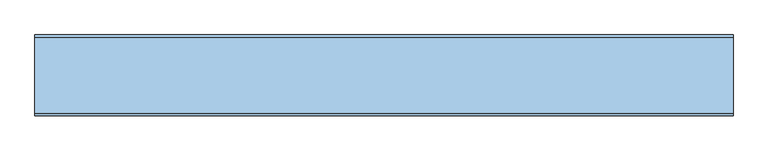
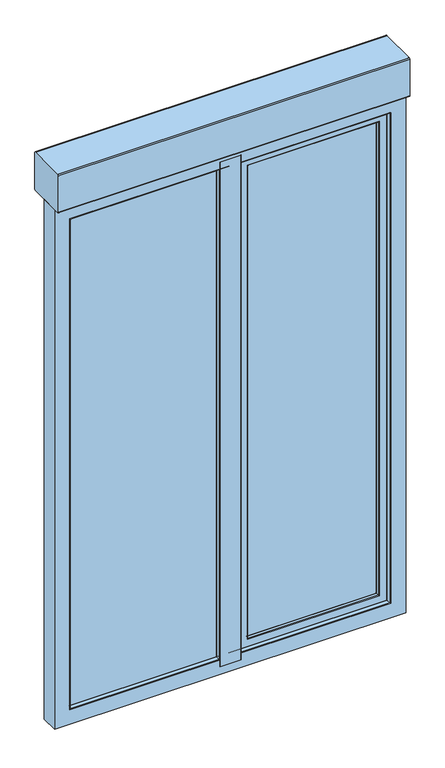
"""IFC4 building model written with IfcOpenShell, lengths in millimetres: window geometry, 2019_ES_Ventana_Replus_re80pvc301_11103_box_1-Hoja_Panel-Fijo-Lateral_con-Compacto : Ventana Sala Oeste."""

from ifc_helpers import new_model, si_unit, point, frame, frame_2d, origin, place, context, project, spatial, polyline, circle_curve, ellipse_curve, trimmed, segment, composite_curve, outline, extrude, source, transform, mapped, element, save
from ifc_brep_helpers import plane_surface, cylinder_surface, advanced_brep


def window_1332a1be(model_context):
    return source(origin(), model_context, "Body", "SolidModel", [
        extrude(outline(composite_curve([segment(trimmed(circle_curve(frame_2d((-55.0, 3315.0)), 5.0), [point((-55.0, 3310.0))], [point((-60.0, 3315.0))], False, "CARTESIAN"), True, "CONTINUOUS"), segment(polyline([(-60.0, 3315.0), (-60.0, 3490.0)]), True, "CONTINUOUS"), segment(trimmed(circle_curve(frame_2d((-55.0, 3490.0)), 5.0), [point((-60.0, 3490.0))], [point((-55.0, 3495.0))], False, "CARTESIAN"), True, "CONTINUOUS"), segment(polyline([(-55.0, 3495.0), (120.0, 3495.0)]), True, "CONTINUOUS"), segment(trimmed(circle_curve(frame_2d((120.0, 3490.0)), 5.0), [point((120.0, 3495.0))], [point((125.0, 3490.0))], False, "CARTESIAN"), True, "CONTINUOUS"), segment(polyline([(125.0, 3490.0), (125.0, 3315.0)]), True, "CONTINUOUS"), segment(trimmed(circle_curve(frame_2d((120.0, 3315.0)), 5.0), [point((125.0, 3315.0))], [point((120.0, 3310.0))], False, "CARTESIAN"), True, "CONTINUOUS"), segment(polyline([(120.0, 3310.0), (-55.0, 3310.0)]), True, "CONTINUOUS")], self_intersect=False)), frame((-800.0, 0.0, 0.0), z_axis=(1.0, 0.0, 0.0), x_axis=(0.0, 1.0, 0.0)), (0.0, 0.0, 1.0), 1600.0),
        extrude(outline(polyline([(78.4999991, 1470.0), (118.4999991, 1470.0), (118.4999991, 1360.0), (98.4999991, 1360.0), (98.4999991, 1450.0), (78.4999991, 1450.0), (78.4999991, 1470.0)])), frame((38.5, 0.0, 0.0), z_axis=(1.0, 0.0, 0.0), x_axis=(0.0, 1.0, 0.0)), (0.0, 0.0, 1.0), 12.0),
        extrude(outline(polyline([(58.7312385, 78.4999991), (58.7312385, 68.4999991), (30.2687615, 68.4999991), (30.2687615, 78.4999991), (58.7312385, 78.4999991)])), frame((0.0, 0.0, 1435.217127), z_axis=(0.0, 0.0, 1.0), x_axis=(1.0, 0.0, 0.0)), (0.0, 0.0, 1.0), 49.565746),
        extrude(outline(polyline([(-37.0063666, -11.4999962), (-734.1891471, -11.4999962), (-734.1891471, -7.4999962), (-37.0063666, -7.4999962), (-37.0063666, -11.4999962)])), frame((0.0, 0.0, 875.6108529), z_axis=(0.0, 0.0, 1.0), x_axis=(1.0, 0.0, 0.0)), (0.0, 0.0, 1.0), 2368.7782941),
        extrude(outline(polyline([(-37.0063666, 6.5), (-734.1891471, 6.5), (-734.1891471, 10.5), (-37.0063666, 10.5), (-37.0063666, 6.5)])), frame((0.0, 0.0, 875.6108529), z_axis=(0.0, 0.0, 1.0), x_axis=(1.0, 0.0, 0.0)), (0.0, 0.0, 1.0), 2368.7782941),
        extrude(outline(polyline([(-37.0063666, 24.4999997), (-734.1891471, 24.4999997), (-734.1891471, 28.4999997), (-37.0063666, 28.4999997), (-37.0063666, 24.4999997)])), frame((0.0, 0.0, 875.6108529), z_axis=(0.0, 0.0, 1.0), x_axis=(1.0, 0.0, 0.0)), (0.0, 0.0, 1.0), 2368.7782941),
        advanced_brep(
        [(-22.1502489, 49.9816666, 3264.0497511), (-22.1502489, 49.9816666, 855.9502489), (-41.8192398, 49.2838062, 875.6192398), (-41.8192398, 49.2838062, 3244.3807602), (-46.4697163, 45.5846502, 880.2697163), (-46.4697163, 45.5846502, 3239.7302837), (-754.0497503, 49.9816666, 855.9502489), (-734.3807594, 49.2838062, 875.6192398), (-21.0, 48.871505, 3265.2), (-21.0, 48.871505, 854.8), (-51.0475336, 28.5000036, 884.8475336), (-51.0475336, 28.5000036, 3235.1524664), (-729.7302829, 45.5846502, 880.2697163), (-43.2922784, 28.5000036, 877.0922784), (-43.2922784, 28.5000036, 3242.9077216), (-732.9077208, 28.5000036, 3242.9077216), (-732.9077208, 28.5000036, 877.0922784), (-725.1524657, 28.5000036, 884.8475336), (-725.1524657, 28.5000036, 3235.1524664), (-35.4855, 36.306782, 869.2855), (-35.4855, 36.306782, 3250.7145), (-35.4855, 39.5069121, 869.2855), (-35.4855, 39.5069121, 3250.7145), (-740.7144993, 36.306782, 869.2855), (-21.0, 39.5069121, 854.8), (-21.0, 39.5069121, 3265.2), (-755.1999993, 39.5069121, 3265.2), (-755.1999993, 39.5069121, 854.8), (-740.7144993, 39.5069121, 869.2855), (-740.7144993, 39.5069121, 3250.7145), (-755.1999993, 48.871505, 854.8), (-754.0497503, 49.9816666, 3264.0497511), (-734.3807594, 49.2838062, 3244.3807602), (-729.7302829, 45.5846502, 3239.7302837), (-740.7144993, 36.306782, 3250.7145), (-755.1999993, 48.871505, 3265.2)],
        [
            (0, 1),
            (1, 2),
            (2, 3),
            (3, 0),
            (2, 4, ellipse_curve(frame((-41.6449168, 44.2918491, 875.4449168), z_axis=(0.7071067811865475, 0.0, 0.7071067811865475), x_axis=(-0.7071067811865474, 0.0, 0.7071067811865476)), 7.0639967, 4.995)),
            (4, 5),
            (5, 3, ellipse_curve(frame((-41.6449168, 44.2918491, 3244.5550832), z_axis=(0.7071067811865475, 0.0, -0.7071067811865475), x_axis=(0.7071067811865474, 0.0, 0.7071067811865476)), 7.0639967, 4.995)),
            (1, 6),
            (6, 7),
            (7, 2),
            (8, 9),
            (9, 1, ellipse_curve(frame((-22.1108601, 48.871505, 855.9108601), z_axis=(0.7071067811865475, 0.0, 0.7071067811865475), x_axis=(-0.7071067811865474, 0.0, 0.7071067811865476)), 1.5709935, 1.1108601)),
            (0, 8, ellipse_curve(frame((-22.1108601, 48.871505, 3264.0891399), z_axis=(0.7071067811865475, 0.0, -0.7071067811865475), x_axis=(0.7071067811865474, 0.0, 0.7071067811865476)), 1.5709935, 1.1108601)),
            (4, 10),
            (10, 11),
            (11, 5),
            (7, 12, ellipse_curve(frame((-734.5550824, 44.2918491, 875.4449168), z_axis=(0.7071067811865475, 0.0, -0.7071067811865475), x_axis=(0.7071067811865476, 0.0, 0.7071067811865474)), 7.0639967, 4.995)),
            (12, 4),
            (13, 14),
            (14, 15),
            (15, 16),
            (16, 13),
            (10, 17),
            (17, 18),
            (18, 11),
            (12, 17),
            (13, 19),
            (19, 20),
            (20, 14),
            (19, 21),
            (21, 22),
            (22, 20),
            (16, 23),
            (23, 19),
            (24, 25),
            (25, 26),
            (26, 27),
            (27, 24),
            (21, 28),
            (28, 29),
            (29, 22),
            (23, 28),
            (8, 25),
            (24, 9),
            (27, 30),
            (30, 9),
            (30, 6, ellipse_curve(frame((-754.0891391, 48.871505, 855.9108601), z_axis=(0.7071067811865475, 0.0, -0.7071067811865475), x_axis=(0.7071067811865476, 0.0, 0.7071067811865474)), 1.5709935, 1.1108601)),
            (6, 31),
            (31, 32),
            (32, 7),
            (32, 33, ellipse_curve(frame((-734.5550824, 44.2918491, 3244.5550832), z_axis=(-0.7071067811865475, 0.0, -0.7071067811865475), x_axis=(0.7071067811865474, 0.0, -0.7071067811865476)), 7.0639967, 4.995)),
            (33, 12),
            (33, 18),
            (15, 34),
            (34, 23),
            (34, 29),
            (26, 35),
            (35, 30),
            (35, 31, ellipse_curve(frame((-754.0891391, 48.871505, 3264.0891399), z_axis=(-0.7071067811865475, 0.0, -0.7071067811865475), x_axis=(0.7071067811865474, 0.0, -0.7071067811865476)), 1.5709935, 1.1108601)),
            (31, 0),
            (3, 32),
            (5, 33),
            (20, 34),
            (8, 35),
        ],
        [
            plane_surface(frame((-41.8192398, 49.2838062, 3244.3807602), z_axis=(-0.03545791932093311, 0.9993711702652975, 0.0), x_axis=(0.0, 0.0, -1.0))),
            cylinder_surface(frame((-41.6449168, 44.2918491, 3272.2), z_axis=(0.0, 0.0, 1.0), x_axis=(-1.0, 0.0, 0.0)), 4.995),
            plane_surface(frame((-41.8192398, 49.2838062, 875.6192398), z_axis=(0.0, 0.9993711702652976, 0.035457919320929884), x_axis=(-1.0, 0.0, 0.0))),
            cylinder_surface(frame((-22.1108601, 48.871505, 3272.2), z_axis=(0.0, 0.0, 1.0), x_axis=(-1.0, 0.0, 0.0)), 1.1108601),
            plane_surface(frame((-51.0475336, 28.5000036, 3235.1524664), z_axis=(-0.9659258262890619, 0.25881904510254483, 0.0), x_axis=(0.0, 0.0, -1.0))),
            cylinder_surface(frame((-14.0, 44.2918491, 875.4449168), z_axis=(1.0, 0.0, 0.0), x_axis=(0.0, 0.0, 1.0)), 4.995),
            plane_surface(frame((-732.9077208, 28.5000036, 3242.9077216), z_axis=(0.0, -1.0, 0.0), x_axis=(1.0, 0.0, 0.0))),
            plane_surface(frame((-51.0475336, 28.5000036, 884.8475336), z_axis=(0.0, 0.25881904510254794, 0.965925826289061), x_axis=(-1.0, 0.0, 0.0))),
            plane_surface(frame((-35.4855, 36.306782, 3250.7145), z_axis=(0.7071067811865617, -0.7071067811865334, 0.0), x_axis=(0.0, 0.0, -1.0))),
            plane_surface(frame((-35.4855, 39.5069121, 3250.7145), z_axis=(1.0, 0.0, 0.0), x_axis=(0.0, 0.0, -1.0))),
            plane_surface(frame((-35.4855, 36.306782, 869.2855), z_axis=(0.0, -0.7071067811865357, -0.7071067811865593), x_axis=(-1.0, 0.0, 0.0))),
            plane_surface(frame((-755.1999993, 39.5069121, 3265.2), z_axis=(0.0, -1.0, 0.0), x_axis=(1.0, 0.0, 0.0))),
            plane_surface(frame((-35.4855, 39.5069121, 869.2855), z_axis=(0.0, 0.0, -1.0), x_axis=(-1.0, 0.0, 0.0))),
            plane_surface(frame((-21.0, 46.2002121, 3265.2), z_axis=(1.0, 0.0, 0.0), x_axis=(0.0, 0.0, -1.0))),
            plane_surface(frame((-21.0, 46.2002121, 854.8), z_axis=(0.0, 0.0, -1.0), x_axis=(-1.0, 0.0, 0.0))),
            cylinder_surface(frame((-14.0, 48.871505, 855.9108601), z_axis=(1.0, 0.0, 0.0), x_axis=(0.0, 0.0, 1.0)), 1.1108601),
            plane_surface(frame((-734.3807594, 49.2838062, 875.6192398), z_axis=(0.03545791932092666, 0.9993711702652978, 0.0), x_axis=(0.0, 0.0, 1.0))),
            cylinder_surface(frame((-734.5550824, 44.2918491, 847.8), z_axis=(0.0, 0.0, -1.0), x_axis=(1.0, 0.0, 0.0)), 4.995),
            plane_surface(frame((-725.1524657, 28.5000036, 884.8475336), z_axis=(0.9659258262890602, 0.2588190451025511, 0.0), x_axis=(0.0, 0.0, 1.0))),
            plane_surface(frame((-740.7144993, 36.306782, 869.2855), z_axis=(-0.707106781186557, -0.707106781186538, 0.0), x_axis=(0.0, 0.0, 1.0))),
            plane_surface(frame((-740.7144993, 39.5069121, 869.2855), z_axis=(-1.0, 0.0, 0.0), x_axis=(0.0, 0.0, 1.0))),
            plane_surface(frame((-755.1999993, 46.2002121, 854.8), z_axis=(-1.0, 0.0, 0.0), x_axis=(0.0, 0.0, 1.0))),
            cylinder_surface(frame((-754.0891391, 48.871505, 847.8), z_axis=(0.0, 0.0, -1.0), x_axis=(1.0, 0.0, 0.0)), 1.1108601),
            plane_surface(frame((-734.3807594, 49.2838062, 3244.3807602), z_axis=(0.0, 0.9993711702652976, -0.035457919320929884), x_axis=(1.0, 0.0, 0.0))),
            cylinder_surface(frame((-762.1999993, 44.2918491, 3244.5550832), z_axis=(-1.0, 0.0, 0.0), x_axis=(0.0, 0.0, -1.0)), 4.995),
            plane_surface(frame((-725.1524657, 28.5000036, 3235.1524664), z_axis=(0.0, 0.258819045102548, -0.9659258262890611), x_axis=(1.0, 0.0, 0.0))),
            plane_surface(frame((-740.7144993, 36.306782, 3250.7145), z_axis=(0.0, -0.7071067811865357, 0.7071067811865593), x_axis=(1.0, 0.0, 0.0))),
            plane_surface(frame((-740.7144993, 39.5069121, 3250.7145), z_axis=(0.0, 0.0, 1.0), x_axis=(1.0, 0.0, 0.0))),
            plane_surface(frame((-755.1999993, 46.2002121, 3265.2), z_axis=(0.0, 0.0, 1.0), x_axis=(1.0, 0.0, 0.0))),
            cylinder_surface(frame((-762.1999993, 48.871505, 3264.0891399), z_axis=(-1.0, 0.0, 0.0), x_axis=(0.0, 0.0, -1.0)), 1.1108601),
        ],
        [
            (0, [[1, 2, 3, 4]]),
            (1, [[-3, 5, 6, 7]]),
            (2, [[8, 9, 10, -2]]),
            (3, [[11, 12, -1, 13]]),
            (4, [[-6, 14, 15, 16]]),
            (5, [[-10, 17, 18, -5]]),
            (6, [[19, 20, 21, 22], [-15, 23, 24, 25]]),
            (7, [[-18, 26, -23, -14]]),
            (8, [[-19, 27, 28, 29]]),
            (9, [[-28, 30, 31, 32]]),
            (10, [[-22, 33, 34, -27]]),
            (11, [[35, 36, 37, 38], [-31, 39, 40, 41]]),
            (12, [[-34, 42, -39, -30]]),
            (13, [[43, -35, 44, -11]]),
            (14, [[-38, 45, 46, -44]]),
            (15, [[-46, 47, -8, -12]]),
            (16, [[48, 49, 50, -9]]),
            (17, [[-50, 51, 52, -17]]),
            (18, [[-52, 53, -24, -26]]),
            (19, [[-21, 54, 55, -33]]),
            (20, [[-55, 56, -40, -42]]),
            (21, [[-37, 57, 58, -45]]),
            (22, [[-58, 59, -48, -47]]),
            (23, [[60, -4, 61, -49]]),
            (24, [[-61, -7, 62, -51]]),
            (25, [[-62, -16, -25, -53]]),
            (26, [[-20, -29, 63, -54]]),
            (27, [[-63, -32, -41, -56]]),
            (28, [[-36, -43, 64, -57]]),
            (29, [[-64, -13, -60, -59]]),
        ],
    ),
        extrude(outline(polyline([(912.8, 697.1999993), (3207.0, 697.1999993), (3207.0, 81.0), (912.8, 81.0), (912.8, 697.1999993)]), holes=[polyline([(3199.0, 689.1999993), (920.8, 689.1999993), (920.8, 89.0), (3199.0, 89.0), (3199.0, 689.1999993)])]), frame((0.0, 11.0, 0.0), z_axis=(0.0, 1.0, 0.0), x_axis=(0.0, 0.0, 1.0)), (0.0, 0.0, 1.0), 16.0000002),
        extrude(outline(polyline([(912.8, 697.1999993), (3207.0, 697.1999993), (3207.0, 81.0), (912.8, 81.0), (912.8, 697.1999993)]), holes=[polyline([(3199.0, 689.1999993), (920.8, 689.1999993), (920.8, 89.0), (3199.0, 89.0), (3199.0, 689.1999993)])]), frame((0.0, 31.0, 0.0), z_axis=(0.0, 1.0, 0.0), x_axis=(0.0, 0.0, 1.0)), (0.0, 0.0, 1.0), 16.0000002),
        extrude(outline(polyline([(881.8608529, -43.0063666), (3238.3891471, -43.0063666), (3238.3891471, -728.1891471), (881.8608529, -728.1891471), (881.8608529, -43.0063666)]), holes=[polyline([(3230.3891471, -51.0063666), (889.8608529, -51.0063666), (889.8608529, -720.1891471), (3230.3891471, -720.1891471), (3230.3891471, -51.0063666)])]), frame((0.0, 10.5, 0.0), z_axis=(0.0, 1.0, 0.0), x_axis=(0.0, 0.0, 1.0)), (0.0, 0.0, 1.0), 14.0),
        extrude(outline(polyline([(881.8608529, -43.0063666), (3238.3891471, -43.0063666), (3238.3891471, -728.1891471), (881.8608529, -728.1891471), (881.8608529, -43.0063666)]), holes=[polyline([(3230.3891471, -51.0063666), (889.8608529, -51.0063666), (889.8608529, -720.1891471), (3230.3891471, -720.1891471), (3230.3891471, -51.0063666)])]), frame((0.0, -7.5, 0.0), z_axis=(0.0, 1.0, 0.0), x_axis=(0.0, 0.0, 1.0)), (0.0, 0.0, 1.0), 14.0),
        advanced_brep(
        [(48.1911809, -11.5, 3240.2), (48.1911809, 11.9999991, 3240.2), (48.1911809, 11.9999991, 879.8), (48.1911809, -11.5, 879.8), (730.1999993, -11.5, 879.8), (730.1999993, -11.5, 3240.2), (88.2020856, -11.5, 919.8109047), (88.2020856, -11.5, 3200.1890953), (690.1890945, -11.5, 3200.1890953), (690.1890945, -11.5, 919.8109047), (730.1999993, 11.9999991, 879.8), (35.1911809, 11.9999991, 3253.2), (35.1911809, 11.9999991, 866.8), (743.1999993, 11.9999991, 866.8), (743.1999993, 11.9999991, 3253.2), (730.1999993, 11.9999991, 3240.2), (35.1911809, 50.0, 3253.2), (35.1911809, 50.0, 866.8), (743.1999993, 50.0, 866.8), (15.1911809, 50.0, 3273.2), (15.1911809, 50.0, 846.8), (763.1999993, 50.0, 846.8), (763.1999993, 50.0, 3273.2), (743.1999993, 50.0, 3253.2), (15.1911809, 65.4999991, 3273.2), (15.1911809, 65.4999991, 846.8), (763.1999993, 65.4999991, 846.8), (18.1911809, 68.4999991, 3270.2), (18.1911809, 68.4999991, 849.8), (760.1999993, 68.4999991, 849.8), (760.1999993, 68.4999991, 3270.2), (70.9541209, 68.4999991, 3217.43706), (70.9541209, 68.4999991, 902.56294), (707.4370593, 68.4999991, 902.56294), (707.4370593, 68.4999991, 3217.43706), (72.1911809, 67.2629391, 3216.2), (72.1911809, 67.2629391, 903.8), (706.1999993, 67.2629391, 903.8), (72.7423375, 67.7951848, 3215.6488434), (72.7423375, 67.7951848, 904.3511566), (705.6488427, 67.7951848, 904.3511566), (85.7676831, 67.3403297, 3202.6234978), (85.7676831, 67.3403297, 917.3765022), (692.6234971, 67.3403297, 917.3765022), (89.4917884, 64.3780426, 3198.8993925), (89.4917884, 64.3780426, 921.1006075), (688.8993918, 64.3780426, 921.1006075), (92.8970803, 51.6693201, 3195.4941006), (92.8970803, 51.6693201, 924.5058994), (685.4940999, 51.6693201, 924.5058994), (92.3834932, 51.0000003, 3196.0076877), (92.3834932, 51.0000003, 923.9923123), (686.007687, 51.0000003, 923.9923123), (81.1911809, 51.0000003, 3207.2), (81.1911809, 51.0000003, 912.8), (697.1999993, 51.0000003, 912.8), (697.1999993, 51.0000003, 3207.2), (686.007687, 51.0000003, 3196.0076877), (81.1911809, 56.4999995, 3207.2), (81.1911809, 56.4999995, 912.8), (697.1999993, 56.4999995, 912.8), (69.1911809, 56.4999995, 3219.2), (69.1911809, 56.4999995, 900.8), (709.1999993, 56.4999995, 900.8), (709.1999993, 56.4999995, 3219.2), (697.1999993, 56.4999995, 3207.2), (69.1911809, 25.6153717, 3219.2), (69.1911809, 25.6153717, 900.8), (709.1999993, 25.6153717, 900.8), (66.574961, 6.9999997, 3221.8162199), (66.574961, 6.9999997, 898.1837801), (711.8162192, 6.9999997, 898.1837801), (711.8162192, 6.9999997, 3221.8162199), (87.1911809, 6.9999997, 3201.2), (87.1911809, 6.9999997, 918.8), (691.1999993, 6.9999997, 918.8), (691.1999993, 6.9999997, 3201.2), (87.1911809, 3.0000033, 3201.2), (87.1911809, 3.0000033, 918.8), (691.1999993, 3.0000033, 918.8), (691.1999993, 3.0000033, 3201.2), (93.7172496, 3.0000033, 3194.6739313), (93.7172496, 3.0000033, 925.3260687), (684.6739305, 3.0000033, 925.3260687), (684.6739305, 3.0000033, 3194.6739313), (94.2153834, 2.3508228, 3194.1757976), (94.2153834, 2.3508228, 925.8242024), (684.1757968, 2.3508228, 925.8242024), (91.0998631, -9.2764571, 3197.2913178), (91.0998631, -9.2764571, 922.7086822), (687.2913171, -9.2764571, 922.7086822), (763.1999993, 65.4999991, 3273.2), (706.1999993, 67.2629391, 3216.2), (705.6488427, 67.7951848, 3215.6488434), (692.6234971, 67.3403297, 3202.6234978), (688.8993918, 64.3780426, 3198.8993925), (685.4940999, 51.6693201, 3195.4941006), (709.1999993, 25.6153717, 3219.2), (684.1757968, 2.3508228, 3194.1757976), (687.2913171, -9.2764571, 3197.2913178)],
        [
            (0, 1),
            (1, 2),
            (2, 3),
            (3, 0),
            (3, 4),
            (4, 5),
            (5, 0),
            (6, 7),
            (7, 8),
            (8, 9),
            (9, 6),
            (2, 10),
            (10, 4),
            (11, 12),
            (12, 13),
            (13, 14),
            (14, 11),
            (1, 15),
            (15, 10),
            (11, 16),
            (16, 17),
            (17, 12),
            (17, 18),
            (18, 13),
            (19, 20),
            (20, 21),
            (21, 22),
            (22, 19),
            (16, 23),
            (23, 18),
            (24, 25),
            (25, 20),
            (19, 24),
            (25, 26),
            (26, 21),
            (27, 28),
            (28, 25, ellipse_curve(frame((18.1911809, 65.4999991, 849.8), z_axis=(-0.7071067811865475, 0.0, 0.7071067811865475), x_axis=(0.7071067811865474, 0.0, 0.7071067811865476)), 4.2426407, 3.0)),
            (24, 27, ellipse_curve(frame((18.1911809, 65.4999991, 3270.2), z_axis=(-0.7071067811865475, 0.0, -0.7071067811865475), x_axis=(-0.7071067811865474, 0.0, 0.7071067811865476)), 4.2426407, 3.0)),
            (28, 29),
            (29, 26, ellipse_curve(frame((760.1999993, 65.4999991, 849.8), z_axis=(-0.7071067811865475, 0.0, -0.7071067811865475), x_axis=(-0.7071067811865476, 0.0, 0.7071067811865474)), 4.2426407, 3.0)),
            (27, 30),
            (30, 29),
            (31, 32),
            (32, 33),
            (33, 34),
            (34, 31),
            (35, 36),
            (36, 32, ellipse_curve(frame((70.9541209, 67.2629391, 902.56294), z_axis=(-0.7071067811865475, 0.0, 0.7071067811865475), x_axis=(0.7071067811865474, 0.0, 0.7071067811865476)), 1.7494671, 1.23706)),
            (31, 35, ellipse_curve(frame((70.9541209, 67.2629391, 3217.43706), z_axis=(-0.7071067811865475, 0.0, -0.7071067811865475), x_axis=(-0.7071067811865474, 0.0, 0.7071067811865476)), 1.7494671, 1.23706)),
            (36, 37),
            (37, 33, ellipse_curve(frame((707.4370593, 67.2629391, 902.56294), z_axis=(-0.7071067811865475, 0.0, -0.7071067811865475), x_axis=(-0.7071067811865476, 0.0, 0.7071067811865474)), 1.7494671, 1.23706)),
            (38, 39),
            (39, 36, ellipse_curve(frame((72.7237511, 67.2629391, 904.3325701), z_axis=(-0.7071067811865475, 0.0, 0.7071067811865475), x_axis=(0.7071067811865474, 0.0, 0.7071067811865476)), 0.7531679, 0.5325701)),
            (35, 38, ellipse_curve(frame((72.7237511, 67.2629391, 3215.6674299), z_axis=(-0.7071067811865475, 0.0, -0.7071067811865475), x_axis=(-0.7071067811865474, 0.0, 0.7071067811865476)), 0.7531679, 0.5325701)),
            (39, 40),
            (40, 37, ellipse_curve(frame((705.6674291, 67.2629391, 904.3325701), z_axis=(-0.7071067811865475, 0.0, -0.7071067811865475), x_axis=(-0.7071067811865476, 0.0, 0.7071067811865474)), 0.7531679, 0.5325701)),
            (41, 42),
            (42, 39),
            (38, 41),
            (42, 43),
            (43, 40),
            (44, 45),
            (45, 42, ellipse_curve(frame((85.6280851, 63.3427664, 917.2369042), z_axis=(-0.7071067811865475, 0.0, 0.7071067811865475), x_axis=(0.7071067811865474, 0.0, 0.7071067811865476)), 5.6568542, 4.0)),
            (41, 44, ellipse_curve(frame((85.6280851, 63.3427664, 3202.7630958), z_axis=(-0.7071067811865475, 0.0, -0.7071067811865475), x_axis=(-0.7071067811865474, 0.0, 0.7071067811865476)), 5.6568542, 4.0)),
            (45, 46),
            (46, 43, ellipse_curve(frame((692.7630951, 63.3427664, 917.2369042), z_axis=(-0.7071067811865475, 0.0, -0.7071067811865475), x_axis=(-0.7071067811865476, 0.0, 0.7071067811865474)), 5.6568542, 4.0)),
            (47, 48),
            (48, 45),
            (44, 47),
            (48, 49),
            (49, 46),
            (50, 51),
            (51, 48, ellipse_curve(frame((92.3834932, 51.5317048, 923.9923123), z_axis=(-0.7071067811865475, 0.0, 0.7071067811865475), x_axis=(0.7071067811865474, 0.0, 0.7071067811865476)), 0.7519437, 0.5317045)),
            (47, 50, ellipse_curve(frame((92.3834932, 51.5317048, 3196.0076877), z_axis=(-0.7071067811865475, 0.0, -0.7071067811865475), x_axis=(-0.7071067811865474, 0.0, 0.7071067811865476)), 0.7519437, 0.5317045)),
            (51, 52),
            (52, 49, ellipse_curve(frame((686.007687, 51.5317048, 923.9923123), z_axis=(-0.7071067811865475, 0.0, -0.7071067811865475), x_axis=(-0.7071067811865476, 0.0, 0.7071067811865474)), 0.7519437, 0.5317045)),
            (53, 54),
            (54, 55),
            (55, 56),
            (56, 53),
            (50, 57),
            (57, 52),
            (58, 59),
            (59, 54),
            (53, 58),
            (59, 60),
            (60, 55),
            (61, 62),
            (62, 63),
            (63, 64),
            (64, 61),
            (58, 65),
            (65, 60),
            (66, 67),
            (67, 62),
            (61, 66),
            (67, 68),
            (68, 63),
            (69, 70),
            (70, 67),
            (66, 69),
            (70, 71),
            (71, 68),
            (69, 72),
            (72, 71),
            (73, 74),
            (74, 75),
            (75, 76),
            (76, 73),
            (77, 78),
            (78, 74),
            (73, 77),
            (78, 79),
            (79, 75),
            (77, 80),
            (80, 79),
            (81, 82),
            (82, 83),
            (83, 84),
            (84, 81),
            (85, 86),
            (86, 82, ellipse_curve(frame((93.7172496, 2.4842973, 925.3260687), z_axis=(-0.7071067811865475, 0.0, 0.7071067811865475), x_axis=(0.7071067811865474, 0.0, 0.7071067811865476)), 0.7293184, 0.515706)),
            (81, 85, ellipse_curve(frame((93.7172496, 2.4842973, 3194.6739313), z_axis=(-0.7071067811865475, 0.0, -0.7071067811865475), x_axis=(-0.7071067811865474, 0.0, 0.7071067811865476)), 0.7293184, 0.515706)),
            (86, 87),
            (87, 83, ellipse_curve(frame((684.6739305, 2.4842973, 925.3260687), z_axis=(-0.7071067811865475, 0.0, -0.7071067811865475), x_axis=(-0.7071067811865476, 0.0, 0.7071067811865474)), 0.7293184, 0.515706)),
            (88, 89),
            (89, 86),
            (85, 88),
            (89, 90),
            (90, 87),
            (6, 89, ellipse_curve(frame((88.2020856, -8.5, 919.8109047), z_axis=(-0.7071067811865475, 0.0, 0.7071067811865475), x_axis=(0.7071067811865474, 0.0, 0.7071067811865476)), 4.2426407, 3.0)),
            (88, 7, ellipse_curve(frame((88.2020856, -8.5, 3200.1890953), z_axis=(-0.7071067811865475, 0.0, -0.7071067811865475), x_axis=(-0.7071067811865474, 0.0, 0.7071067811865476)), 4.2426407, 3.0)),
            (9, 90, ellipse_curve(frame((690.1890945, -8.5, 919.8109047), z_axis=(-0.7071067811865475, 0.0, -0.7071067811865475), x_axis=(-0.7071067811865476, 0.0, 0.7071067811865474)), 4.2426407, 3.0)),
            (15, 5),
            (23, 14),
            (26, 91),
            (91, 22),
            (30, 91, ellipse_curve(frame((760.1999993, 65.4999991, 3270.2), z_axis=(0.7071067811865475, 0.0, -0.7071067811865475), x_axis=(-0.7071067811865474, 0.0, -0.7071067811865476)), 4.2426407, 3.0)),
            (37, 92),
            (92, 34, ellipse_curve(frame((707.4370593, 67.2629391, 3217.43706), z_axis=(0.7071067811865475, 0.0, -0.7071067811865475), x_axis=(-0.7071067811865474, 0.0, -0.7071067811865476)), 1.7494671, 1.23706)),
            (40, 93),
            (93, 92, ellipse_curve(frame((705.6674291, 67.2629391, 3215.6674299), z_axis=(0.7071067811865475, 0.0, -0.7071067811865475), x_axis=(-0.7071067811865474, 0.0, -0.7071067811865476)), 0.7531679, 0.5325701)),
            (43, 94),
            (94, 93),
            (46, 95),
            (95, 94, ellipse_curve(frame((692.7630951, 63.3427664, 3202.7630958), z_axis=(0.7071067811865475, 0.0, -0.7071067811865475), x_axis=(-0.7071067811865474, 0.0, -0.7071067811865476)), 5.6568542, 4.0)),
            (49, 96),
            (96, 95),
            (57, 96, ellipse_curve(frame((686.007687, 51.5317048, 3196.0076877), z_axis=(0.7071067811865475, 0.0, -0.7071067811865475), x_axis=(-0.7071067811865474, 0.0, -0.7071067811865476)), 0.7519437, 0.5317045)),
            (65, 56),
            (68, 97),
            (97, 64),
            (72, 97),
            (80, 76),
            (87, 98),
            (98, 84, ellipse_curve(frame((684.6739305, 2.4842973, 3194.6739313), z_axis=(0.7071067811865475, 0.0, -0.7071067811865475), x_axis=(-0.7071067811865474, 0.0, -0.7071067811865476)), 0.7293184, 0.515706)),
            (90, 99),
            (99, 98),
            (8, 99, ellipse_curve(frame((690.1890945, -8.5, 3200.1890953), z_axis=(0.7071067811865475, 0.0, -0.7071067811865475), x_axis=(-0.7071067811865474, 0.0, -0.7071067811865476)), 4.2426407, 3.0)),
            (91, 24),
            (92, 35),
            (93, 38),
            (94, 41),
            (95, 44),
            (96, 47),
            (97, 66),
            (98, 85),
            (99, 88),
        ],
        [
            plane_surface(frame((48.1911809, 1.4999991, 3240.2), z_axis=(-1.0, 0.0, 0.0), x_axis=(0.0, 0.0, -1.0))),
            plane_surface(frame((690.1890945, -11.5, 3200.1890953), z_axis=(0.0, -1.0, 0.0), x_axis=(-1.0, 0.0, 0.0))),
            plane_surface(frame((48.1911809, 1.4999991, 879.8), z_axis=(0.0, 0.0, -1.0), x_axis=(1.0, 0.0, 0.0))),
            plane_surface(frame((735.7000002, 11.9999991, 3245.7000009), z_axis=(0.0, -1.0, 0.0), x_axis=(-1.0, 0.0, 0.0))),
            plane_surface(frame((35.1911809, 45.0999991, 3253.2), z_axis=(-1.0, 0.0, 0.0), x_axis=(0.0, 0.0, -1.0))),
            plane_surface(frame((35.1911809, 45.0999991, 866.8), z_axis=(0.0, 0.0, -1.0), x_axis=(1.0, 0.0, 0.0))),
            plane_surface(frame((759.2000019, 50.0, 3269.2000027), z_axis=(0.0, -1.0, 0.0), x_axis=(-1.0, 0.0, 0.0))),
            plane_surface(frame((15.1911809, 50.0, 3273.2), z_axis=(-1.0, 0.0, 0.0), x_axis=(0.0, 0.0, -1.0))),
            plane_surface(frame((15.1911809, 50.0, 846.8), z_axis=(0.0, 0.0, -1.0), x_axis=(1.0, 0.0, 0.0))),
            cylinder_surface(frame((18.1911809, 65.4999991, 3273.2), z_axis=(0.0, 0.0, 1.0), x_axis=(0.0, -1.0, 0.0)), 3.0),
            cylinder_surface(frame((15.1911809, 65.4999991, 849.8), z_axis=(-1.0, 0.0, 0.0), x_axis=(0.0, -1.0, 0.0)), 3.0),
            plane_surface(frame((760.1999993, 68.4999991, 3270.2), z_axis=(0.0, 1.0, 0.0), x_axis=(-1.0, 0.0, 0.0))),
            cylinder_surface(frame((70.9541209, 67.2629391, 3273.2), z_axis=(0.0, 0.0, 1.0), x_axis=(0.0, -1.0, 0.0)), 1.23706),
            cylinder_surface(frame((15.1911809, 67.2629391, 902.56294), z_axis=(-1.0, 0.0, 0.0), x_axis=(0.0, -1.0, 0.0)), 1.23706),
            cylinder_surface(frame((72.7237511, 67.2629391, 3273.2), z_axis=(0.0, 0.0, 1.0), x_axis=(0.0, -1.0, 0.0)), 0.5325701),
            cylinder_surface(frame((15.1911809, 67.2629391, 904.3325701), z_axis=(-1.0, 0.0, 0.0), x_axis=(0.0, -1.0, 0.0)), 0.5325701),
            plane_surface(frame((72.7423375, 67.7951848, 3215.6488434), z_axis=(0.03489949670249966, 0.9993908270190959, 0.0), x_axis=(0.0, 0.0, -1.0))),
            plane_surface(frame((72.7423375, 67.7951848, 904.3511566), z_axis=(0.0, 0.9993908270190958, 0.034899496702502884), x_axis=(1.0, 0.0, 0.0))),
            cylinder_surface(frame((85.6280851, 63.3427664, 3273.2), z_axis=(0.0, 0.0, 1.0), x_axis=(0.0, -1.0, 0.0)), 4.0),
            cylinder_surface(frame((15.1911809, 63.3427664, 917.2369042), z_axis=(-1.0, 0.0, 0.0), x_axis=(0.0, -1.0, 0.0)), 4.0),
            plane_surface(frame((89.4917884, 64.3780426, 3198.8993925), z_axis=(0.9659258262890643, 0.2588190451025359, 0.0), x_axis=(0.0, 0.0, -1.0))),
            plane_surface(frame((89.4917884, 64.3780426, 921.1006075), z_axis=(0.0, 0.2588190451025328, 0.9659258262890652), x_axis=(1.0, 0.0, 0.0))),
            cylinder_surface(frame((92.3834932, 51.5317048, 3273.2), z_axis=(0.0, 0.0, 1.0), x_axis=(0.0, -1.0, 0.0)), 0.5317045),
            cylinder_surface(frame((15.1911809, 51.5317048, 923.9923123), z_axis=(-1.0, 0.0, 0.0), x_axis=(0.0, -1.0, 0.0)), 0.5317045),
            plane_surface(frame((686.007687, 51.0000003, 3196.0076877), z_axis=(0.0, -1.0, 0.0), x_axis=(-1.0, 0.0, 0.0))),
            plane_surface(frame((81.1911809, 51.0000003, 3207.2), z_axis=(-1.0, 0.0, 0.0), x_axis=(0.0, 0.0, -1.0))),
            plane_surface(frame((81.1911809, 51.0000003, 912.8), z_axis=(0.0, 0.0, -1.0), x_axis=(1.0, 0.0, 0.0))),
            plane_surface(frame((697.1999993, 56.4999995, 3207.2), z_axis=(0.0, -1.0, 0.0), x_axis=(-1.0, 0.0, 0.0))),
            plane_surface(frame((69.1911809, 56.4999995, 3219.2), z_axis=(1.0, 0.0, 0.0), x_axis=(0.0, 0.0, -1.0))),
            plane_surface(frame((69.1911809, 56.4999995, 900.8), z_axis=(0.0, 0.0, 1.0), x_axis=(1.0, 0.0, 0.0))),
            plane_surface(frame((69.1911809, 25.6153717, 3219.2), z_axis=(0.9902680687415736, -0.13917310096004257, 0.0), x_axis=(0.0, 0.0, -1.0))),
            plane_surface(frame((69.1911809, 25.6153717, 900.8), z_axis=(0.0, -0.13917310096004576, 0.9902680687415731), x_axis=(1.0, 0.0, 0.0))),
            plane_surface(frame((711.8162192, 6.9999997, 3221.8162199), z_axis=(0.0, 1.0, 0.0), x_axis=(-1.0, 0.0, 0.0))),
            plane_surface(frame((87.1911809, 6.9999997, 3201.2), z_axis=(1.0, 0.0, 0.0), x_axis=(0.0, 0.0, -1.0))),
            plane_surface(frame((87.1911809, 6.9999997, 918.8), z_axis=(0.0, 0.0, 1.0), x_axis=(1.0, 0.0, 0.0))),
            plane_surface(frame((691.1999993, 3.0000033, 3201.2), z_axis=(0.0, 1.0, 0.0), x_axis=(-1.0, 0.0, 0.0))),
            cylinder_surface(frame((93.7172496, 2.4842973, 3273.2), z_axis=(0.0, 0.0, 1.0), x_axis=(0.0, -1.0, 0.0)), 0.515706),
            cylinder_surface(frame((15.1911809, 2.4842973, 925.3260687), z_axis=(-1.0, 0.0, 0.0), x_axis=(0.0, -1.0, 0.0)), 0.515706),
            plane_surface(frame((94.2153834, 2.3508228, 3194.1757976), z_axis=(0.9659258263570589, -0.2588190448487762, 0.0), x_axis=(0.0, 0.0, -1.0))),
            plane_surface(frame((94.2153834, 2.3508228, 925.8242024), z_axis=(0.0, -0.2588190448487794, 0.9659258263570581), x_axis=(1.0, 0.0, 0.0))),
            cylinder_surface(frame((88.2020856, -8.5, 3273.2), z_axis=(0.0, 0.0, 1.0), x_axis=(0.0, -1.0, 0.0)), 3.0),
            cylinder_surface(frame((15.1911809, -8.5, 919.8109047), z_axis=(-1.0, 0.0, 0.0), x_axis=(0.0, -1.0, 0.0)), 3.0),
            plane_surface(frame((730.1999993, 1.4999991, 879.8), z_axis=(1.0, 0.0, 0.0), x_axis=(0.0, 0.0, 1.0))),
            plane_surface(frame((743.1999993, 45.0999991, 866.8), z_axis=(1.0, 0.0, 0.0), x_axis=(0.0, 0.0, 1.0))),
            plane_surface(frame((763.1999993, 50.0, 846.8), z_axis=(1.0, 0.0, 0.0), x_axis=(0.0, 0.0, 1.0))),
            cylinder_surface(frame((760.1999993, 65.4999991, 846.8), z_axis=(0.0, 0.0, -1.0), x_axis=(0.0, -1.0, 0.0)), 3.0),
            cylinder_surface(frame((707.4370593, 67.2629391, 846.8), z_axis=(0.0, 0.0, -1.0), x_axis=(0.0, -1.0, 0.0)), 1.23706),
            cylinder_surface(frame((705.6674291, 67.2629391, 846.8), z_axis=(0.0, 0.0, -1.0), x_axis=(0.0, -1.0, 0.0)), 0.5325701),
            plane_surface(frame((705.6488427, 67.7951848, 904.3511566), z_axis=(-0.03489949670250611, 0.9993908270190957, 0.0), x_axis=(0.0, 0.0, 1.0))),
            cylinder_surface(frame((692.7630951, 63.3427664, 846.8), z_axis=(0.0, 0.0, -1.0), x_axis=(0.0, -1.0, 0.0)), 4.0),
            plane_surface(frame((688.8993918, 64.3780426, 921.1006075), z_axis=(-0.965925826289066, 0.2588190451025297, 0.0), x_axis=(0.0, 0.0, 1.0))),
            cylinder_surface(frame((686.007687, 51.5317048, 846.8), z_axis=(0.0, 0.0, -1.0), x_axis=(0.0, -1.0, 0.0)), 0.5317045),
            plane_surface(frame((697.1999993, 51.0000003, 912.8), z_axis=(1.0, 0.0, 0.0), x_axis=(0.0, 0.0, 1.0))),
            plane_surface(frame((709.1999993, 56.4999995, 900.8), z_axis=(-1.0, 0.0, 0.0), x_axis=(0.0, 0.0, 1.0))),
            plane_surface(frame((709.1999993, 25.6153717, 900.8), z_axis=(-0.9902680687415727, -0.13917310096004895, 0.0), x_axis=(0.0, 0.0, 1.0))),
            plane_surface(frame((691.1999993, 6.9999997, 918.8), z_axis=(-1.0, 0.0, 0.0), x_axis=(0.0, 0.0, 1.0))),
            cylinder_surface(frame((684.6739305, 2.4842973, 846.8), z_axis=(0.0, 0.0, -1.0), x_axis=(0.0, -1.0, 0.0)), 0.515706),
            plane_surface(frame((684.1757968, 2.3508228, 925.8242024), z_axis=(-0.9659258263570573, -0.2588190448487825, 0.0), x_axis=(0.0, 0.0, 1.0))),
            cylinder_surface(frame((690.1890945, -8.5, 846.8), z_axis=(0.0, 0.0, -1.0), x_axis=(0.0, -1.0, 0.0)), 3.0),
            plane_surface(frame((730.1999993, 1.4999991, 3240.2), z_axis=(0.0, 0.0, 1.0), x_axis=(-1.0, 0.0, 0.0))),
            plane_surface(frame((743.1999993, 45.0999991, 3253.2), z_axis=(0.0, 0.0, 1.0), x_axis=(-1.0, 0.0, 0.0))),
            plane_surface(frame((763.1999993, 50.0, 3273.2), z_axis=(0.0, 0.0, 1.0), x_axis=(-1.0, 0.0, 0.0))),
            cylinder_surface(frame((763.1999993, 65.4999991, 3270.2), z_axis=(1.0, 0.0, 0.0), x_axis=(0.0, -1.0, 0.0)), 3.0),
            cylinder_surface(frame((763.1999993, 67.2629391, 3217.43706), z_axis=(1.0, 0.0, 0.0), x_axis=(0.0, -1.0, 0.0)), 1.23706),
            cylinder_surface(frame((763.1999993, 67.2629391, 3215.6674299), z_axis=(1.0, 0.0, 0.0), x_axis=(0.0, -1.0, 0.0)), 0.5325701),
            plane_surface(frame((705.6488427, 67.7951848, 3215.6488434), z_axis=(0.0, 0.9993908270190958, -0.034899496702502884), x_axis=(-1.0, 0.0, 0.0))),
            cylinder_surface(frame((763.1999993, 63.3427664, 3202.7630958), z_axis=(1.0, 0.0, 0.0), x_axis=(0.0, -1.0, 0.0)), 4.0),
            plane_surface(frame((688.8993918, 64.3780426, 3198.8993925), z_axis=(0.0, 0.2588190451025328, -0.9659258262890651), x_axis=(-1.0, 0.0, 0.0))),
            cylinder_surface(frame((763.1999993, 51.5317048, 3196.0076877), z_axis=(1.0, 0.0, 0.0), x_axis=(0.0, -1.0, 0.0)), 0.5317045),
            plane_surface(frame((697.1999993, 51.0000003, 3207.2), z_axis=(0.0, 0.0, 1.0), x_axis=(-1.0, 0.0, 0.0))),
            plane_surface(frame((709.1999993, 56.4999995, 3219.2), z_axis=(0.0, 0.0, -1.0), x_axis=(-1.0, 0.0, 0.0))),
            plane_surface(frame((709.1999993, 25.6153717, 3219.2), z_axis=(0.0, -0.13917310096004576, -0.9902680687415731), x_axis=(-1.0, 0.0, 0.0))),
            plane_surface(frame((691.1999993, 6.9999997, 3201.2), z_axis=(0.0, 0.0, -1.0), x_axis=(-1.0, 0.0, 0.0))),
            cylinder_surface(frame((763.1999993, 2.4842973, 3194.6739313), z_axis=(1.0, 0.0, 0.0), x_axis=(0.0, -1.0, 0.0)), 0.515706),
            plane_surface(frame((684.1757968, 2.3508228, 3194.1757976), z_axis=(0.0, -0.2588190448487794, -0.9659258263570581), x_axis=(-1.0, 0.0, 0.0))),
            cylinder_surface(frame((763.1999993, -8.5, 3200.1890953), z_axis=(1.0, 0.0, 0.0), x_axis=(0.0, -1.0, 0.0)), 3.0),
        ],
        [
            (0, [[1, 2, 3, 4]]),
            (1, [[-4, 5, 6, 7], [8, 9, 10, 11]]),
            (2, [[12, 13, -5, -3]]),
            (3, [[14, 15, 16, 17], [-2, 18, 19, -12]]),
            (4, [[20, 21, 22, -14]]),
            (5, [[23, 24, -15, -22]]),
            (6, [[25, 26, 27, 28], [-21, 29, 30, -23]]),
            (7, [[31, 32, -25, 33]]),
            (8, [[34, 35, -26, -32]]),
            (9, [[36, 37, -31, 38]]),
            (10, [[39, 40, -34, -37]]),
            (11, [[-36, 41, 42, -39], [43, 44, 45, 46]]),
            (12, [[47, 48, -43, 49]]),
            (13, [[50, 51, -44, -48]]),
            (14, [[52, 53, -47, 54]]),
            (15, [[55, 56, -50, -53]]),
            (16, [[57, 58, -52, 59]]),
            (17, [[60, 61, -55, -58]]),
            (18, [[62, 63, -57, 64]]),
            (19, [[65, 66, -60, -63]]),
            (20, [[67, 68, -62, 69]]),
            (21, [[70, 71, -65, -68]]),
            (22, [[72, 73, -67, 74]]),
            (23, [[75, 76, -70, -73]]),
            (24, [[77, 78, 79, 80], [-72, 81, 82, -75]]),
            (25, [[83, 84, -77, 85]]),
            (26, [[86, 87, -78, -84]]),
            (27, [[88, 89, 90, 91], [-83, 92, 93, -86]]),
            (28, [[94, 95, -88, 96]]),
            (29, [[97, 98, -89, -95]]),
            (30, [[99, 100, -94, 101]]),
            (31, [[102, 103, -97, -100]]),
            (32, [[-99, 104, 105, -102], [106, 107, 108, 109]]),
            (33, [[110, 111, -106, 112]]),
            (34, [[113, 114, -107, -111]]),
            (35, [[-110, 115, 116, -113], [117, 118, 119, 120]]),
            (36, [[121, 122, -117, 123]]),
            (37, [[124, 125, -118, -122]]),
            (38, [[126, 127, -121, 128]]),
            (39, [[129, 130, -124, -127]]),
            (40, [[-8, 131, -126, 132]]),
            (41, [[-11, 133, -129, -131]]),
            (42, [[-19, 134, -6, -13]]),
            (43, [[-30, 135, -16, -24]]),
            (44, [[136, 137, -27, -35]]),
            (45, [[-42, 138, -136, -40]]),
            (46, [[139, 140, -45, -51]]),
            (47, [[141, 142, -139, -56]]),
            (48, [[143, 144, -141, -61]]),
            (49, [[145, 146, -143, -66]]),
            (50, [[147, 148, -145, -71]]),
            (51, [[-82, 149, -147, -76]]),
            (52, [[-93, 150, -79, -87]]),
            (53, [[151, 152, -90, -98]]),
            (54, [[-105, 153, -151, -103]]),
            (55, [[-116, 154, -108, -114]]),
            (56, [[155, 156, -119, -125]]),
            (57, [[157, 158, -155, -130]]),
            (58, [[-10, 159, -157, -133]]),
            (59, [[-18, -1, -7, -134]]),
            (60, [[-29, -20, -17, -135]]),
            (61, [[160, -33, -28, -137]]),
            (62, [[-41, -38, -160, -138]]),
            (63, [[161, -49, -46, -140]]),
            (64, [[162, -54, -161, -142]]),
            (65, [[163, -59, -162, -144]]),
            (66, [[164, -64, -163, -146]]),
            (67, [[165, -69, -164, -148]]),
            (68, [[-81, -74, -165, -149]]),
            (69, [[-92, -85, -80, -150]]),
            (70, [[166, -96, -91, -152]]),
            (71, [[-104, -101, -166, -153]]),
            (72, [[-115, -112, -109, -154]]),
            (73, [[167, -123, -120, -156]]),
            (74, [[168, -128, -167, -158]]),
            (75, [[-9, -132, -168, -159]]),
        ],
    ),
        extrude(outline(composite_curve([segment(polyline([(23.3911809, 37.9746327), (20.3911809, 37.9746327), (20.3911809, 8.0), (42.4020331, 8.0), (42.4020331, 6.2175904), (29.7799071, -1.0697975), (28.5556588, -15.0630198), (42.8115567, -17.0665556), (43.5938856, -11.4999962), (54.3579009, -11.4999962)]), True, "CONTINUOUS"), segment(trimmed(circle_curve(frame_2d((54.3579009, -12.4999962)), 1.0), [point((54.3579009, -11.4999962))], [point((55.3238267, -12.7588152))], False, "CARTESIAN"), True, "CONTINUOUS"), segment(polyline([(55.3238267, -12.7588152), (51.2998617, -27.7764571)]), True, "CONTINUOUS"), segment(trimmed(circle_curve(frame_2d((48.4020842, -27.0)), 3.0), [point((51.2998617, -27.7764571))], [point((48.4020842, -30.0))], False, "CARTESIAN"), True, "CONTINUOUS"), segment(polyline([(48.4020842, -30.0), (-46.6020842, -30.0)]), True, "CONTINUOUS"), segment(trimmed(circle_curve(frame_2d((-46.6020842, -27.0)), 3.0), [point((-46.6020842, -30.0))], [point((-49.4998617, -27.7764571))], False, "CARTESIAN"), True, "CONTINUOUS"), segment(polyline([(-49.4998617, -27.7764571), (-53.5238267, -12.7588152)]), True, "CONTINUOUS"), segment(trimmed(circle_curve(frame_2d((-52.5579009, -12.4999962)), 1.0), [point((-53.5238267, -12.7588152))], [point((-52.5579009, -11.4999962))], False, "CARTESIAN"), True, "CONTINUOUS"), segment(polyline([(-52.5579009, -11.4999962), (-41.7938856, -11.4999962), (-41.0115567, -17.0665556), (-26.7556588, -15.0630198), (-27.9799071, -1.0697975), (-40.6020331, 6.2175904), (-40.6020331, 8.0), (-18.5911809, 8.0), (-18.5911809, 37.9746327), (-20.7446784, 37.9746327), (-20.7446784, 49.0)]), True, "CONTINUOUS"), segment(trimmed(circle_curve(frame_2d((-19.7446784, 49.0)), 1.0), [point((-20.7446784, 49.0))], [point((-19.7446784, 50.0))], False, "CARTESIAN"), True, "CONTINUOUS"), segment(polyline([(-19.7446784, 50.0), (22.3911809, 50.0)]), True, "CONTINUOUS"), segment(trimmed(circle_curve(frame_2d((22.3911809, 49.0)), 1.0), [point((22.3911809, 50.0))], [point((23.3911809, 49.0))], False, "CARTESIAN"), True, "CONTINUOUS"), segment(polyline([(23.3911809, 49.0), (23.3911809, 37.9746327)]), True, "CONTINUOUS")], self_intersect=False)), frame((0.0, 0.0, 846.8), z_axis=(0.0, 0.0, 1.0), x_axis=(1.0, 0.0, 0.0)), (0.0, 0.0, 1.0), 2426.4),
        extrude(outline(polyline([(703.1999993, 6.9999997), (75.0, 6.9999997), (75.0, 10.9999997), (703.1999993, 10.9999997), (703.1999993, 6.9999997)])), frame((0.0, 0.0, 906.8), z_axis=(0.0, 0.0, 1.0), x_axis=(1.0, 0.0, 0.0)), (0.0, 0.0, 1.0), 2306.2),
        extrude(outline(polyline([(703.1999993, 26.9999997), (75.0, 26.9999997), (75.0, 30.9999997), (703.1999993, 30.9999997), (703.1999993, 26.9999997)])), frame((0.0, 0.0, 906.8), z_axis=(0.0, 0.0, 1.0), x_axis=(1.0, 0.0, 0.0)), (0.0, 0.0, 1.0), 2306.2),
        extrude(outline(polyline([(703.1999993, 46.9999997), (75.0, 46.9999997), (75.0, 50.9999997), (703.1999993, 50.9999997), (703.1999993, 46.9999997)])), frame((0.0, 0.0, 906.8), z_axis=(0.0, 0.0, 1.0), x_axis=(1.0, 0.0, 0.0)), (0.0, 0.0, 1.0), 2306.2),
        advanced_brep(
        [(756.1999993, 50.0, 3266.1999993), (756.1999993, 50.0, 853.8000007), (755.1999993, 49.0, 854.8000007), (755.1999993, 49.0, 3265.1999993), (755.1999993, 8.0, 854.8000007), (755.1999993, 8.0, 3265.1999993), (-756.1999993, 50.0, 853.8000007), (-755.1999993, 49.0, 854.8000007), (800.0, 50.0, 3310.0), (800.0, 50.0, 810.0), (-800.0, 50.0, 810.0), (-800.0, 50.0, 3310.0), (-756.1999993, 50.0, 3266.1999993), (724.2332803, -11.5, 3234.2332803), (724.2332803, -11.5, 885.7667197), (723.2673545, -12.758819, 886.7326455), (723.2673545, -12.758819, 3233.2673545), (727.2913185, -27.7764571, 882.7086815), (727.2913185, -27.7764571, 3237.2913185), (-724.2332803, -11.5, 885.7667197), (-723.2673545, -12.758819, 886.7326455), (736.1891471, -11.5, 3246.1891471), (736.1891471, -11.5, 873.8108529), (-736.1891471, -11.5, 873.8108529), (-736.1891471, -11.5, 3246.1891471), (-724.2332803, -11.5, 3234.2332803), (730.189096, -30.0, 879.810904), (730.189096, -30.0, 3240.189096), (800.0, -30.0, 810.0), (800.0, -30.0, 3310.0), (-800.0, -30.0, 3310.0), (-800.0, -30.0, 810.0), (-730.189096, -30.0, 879.810904), (-730.189096, -30.0, 3240.189096), (-727.2913185, -27.7764571, 882.7086815), (736.1891471, 8.0, 3246.1891471), (736.1891471, 8.0, 873.8108529), (-736.1891471, 8.0, 873.8108529), (-755.1999993, 8.0, 854.8000007), (-755.1999993, 8.0, 3265.1999993), (-736.1891471, 8.0, 3246.1891471), (-755.1999993, 49.0, 3265.1999993), (-723.2673545, -12.758819, 3233.2673545), (-727.2913185, -27.7764571, 3237.2913185)],
        [
            (0, 1),
            (1, 2, ellipse_curve(frame((756.1999993, 49.0, 853.8000007), z_axis=(0.7071067811865475, 0.0, 0.7071067811865475), x_axis=(-0.7071067811865474, 0.0, 0.7071067811865476)), 1.4142136, 1.0)),
            (2, 3),
            (3, 0, ellipse_curve(frame((756.1999993, 49.0, 3266.1999993), z_axis=(0.7071067811865475, 0.0, -0.7071067811865475), x_axis=(0.7071067811865474, 0.0, 0.7071067811865476)), 1.4142136, 1.0)),
            (2, 4),
            (4, 5),
            (5, 3),
            (1, 6),
            (6, 7, ellipse_curve(frame((-756.1999993, 49.0, 853.8000007), z_axis=(0.7071067811865475, 0.0, -0.7071067811865475), x_axis=(0.7071067811865476, 0.0, 0.7071067811865474)), 1.4142136, 1.0)),
            (7, 2),
            (8, 9),
            (9, 10),
            (10, 11),
            (11, 8),
            (0, 12),
            (12, 6),
            (13, 14),
            (14, 15, ellipse_curve(frame((724.2332803, -12.5, 885.7667197), z_axis=(0.7071067811865475, 0.0, 0.7071067811865475), x_axis=(-0.7071067811865474, 0.0, 0.7071067811865476)), 1.4142136, 1.0)),
            (15, 16),
            (16, 13, ellipse_curve(frame((724.2332803, -12.5, 3234.2332803), z_axis=(0.7071067811865475, 0.0, -0.7071067811865475), x_axis=(0.7071067811865474, 0.0, 0.7071067811865476)), 1.4142136, 1.0)),
            (15, 17),
            (17, 18),
            (18, 16),
            (14, 19),
            (19, 20, ellipse_curve(frame((-724.2332803, -12.5, 885.7667197), z_axis=(0.7071067811865475, 0.0, -0.7071067811865475), x_axis=(0.7071067811865476, 0.0, 0.7071067811865474)), 1.4142136, 1.0)),
            (20, 15),
            (21, 22),
            (22, 23),
            (23, 24),
            (24, 21),
            (13, 25),
            (25, 19),
            (17, 26, ellipse_curve(frame((730.189096, -27.0, 879.810904), z_axis=(0.7071067811865475, 0.0, 0.7071067811865475), x_axis=(-0.7071067811865474, 0.0, 0.7071067811865476)), 4.2426407, 3.0)),
            (26, 27),
            (27, 18, ellipse_curve(frame((730.189096, -27.0, 3240.189096), z_axis=(0.7071067811865475, 0.0, -0.7071067811865475), x_axis=(0.7071067811865474, 0.0, 0.7071067811865476)), 4.2426407, 3.0)),
            (28, 29),
            (29, 30),
            (30, 31),
            (31, 28),
            (26, 32),
            (32, 33),
            (33, 27),
            (17, 34),
            (34, 32, ellipse_curve(frame((-730.189096, -27.0, 879.810904), z_axis=(0.7071067811865475, 0.0, -0.7071067811865475), x_axis=(0.7071067811865476, 0.0, 0.7071067811865474)), 4.2426407, 3.0)),
            (20, 34),
            (35, 36),
            (36, 22),
            (21, 35),
            (36, 37),
            (37, 23),
            (4, 38),
            (38, 39),
            (39, 5),
            (35, 40),
            (40, 37),
            (28, 9),
            (8, 29),
            (31, 10),
            (7, 38),
            (12, 41, ellipse_curve(frame((-756.1999993, 49.0, 3266.1999993), z_axis=(-0.7071067811865475, 0.0, -0.7071067811865475), x_axis=(0.7071067811865474, 0.0, -0.7071067811865476)), 1.4142136, 1.0)),
            (41, 7),
            (25, 42, ellipse_curve(frame((-724.2332803, -12.5, 3234.2332803), z_axis=(-0.7071067811865475, 0.0, -0.7071067811865475), x_axis=(0.7071067811865474, 0.0, -0.7071067811865476)), 1.4142136, 1.0)),
            (42, 20),
            (34, 43),
            (43, 33, ellipse_curve(frame((-730.189096, -27.0, 3240.189096), z_axis=(-0.7071067811865475, 0.0, -0.7071067811865475), x_axis=(0.7071067811865474, 0.0, -0.7071067811865476)), 4.2426407, 3.0)),
            (42, 43),
            (40, 24),
            (30, 11),
            (41, 39),
            (3, 41),
            (16, 42),
            (43, 18),
        ],
        [
            cylinder_surface(frame((756.1999993, 49.0, 3310.0), z_axis=(0.0, 0.0, 1.0), x_axis=(-1.0, 0.0, 0.0)), 1.0),
            plane_surface(frame((755.1999993, 8.0, 3265.1999993), z_axis=(-1.0, 0.0, 0.0), x_axis=(0.0, 0.0, -1.0))),
            cylinder_surface(frame((800.0, 49.0, 853.8000007), z_axis=(1.0, 0.0, 0.0), x_axis=(0.0, 0.0, 1.0)), 1.0),
            plane_surface(frame((-756.1999993, 50.0, 3266.1999993), z_axis=(0.0, 1.0, 0.0), x_axis=(1.0, 0.0, 0.0))),
            cylinder_surface(frame((724.2332803, -12.5, 3310.0), z_axis=(0.0, 0.0, 1.0), x_axis=(-1.0, 0.0, 0.0)), 1.0),
            plane_surface(frame((727.2913185, -27.7764571, 3237.2913185), z_axis=(-0.9659258262890672, -0.25881904510252485, 0.0), x_axis=(0.0, 0.0, -1.0))),
            cylinder_surface(frame((800.0, -12.5, 885.7667197), z_axis=(1.0, 0.0, 0.0), x_axis=(0.0, 0.0, 1.0)), 1.0),
            plane_surface(frame((-724.2332803, -11.5, 3234.2332803), z_axis=(0.0, 1.0, 0.0), x_axis=(1.0, 0.0, 0.0))),
            cylinder_surface(frame((730.189096, -27.0, 3310.0), z_axis=(0.0, 0.0, 1.0), x_axis=(-1.0, 0.0, 0.0)), 3.0),
            plane_surface(frame((-800.0, -30.0, 3310.0), z_axis=(0.0, -1.0, 0.0), x_axis=(1.0, 0.0, 0.0))),
            cylinder_surface(frame((800.0, -27.0, 879.810904), z_axis=(1.0, 0.0, 0.0), x_axis=(0.0, 0.0, 1.0)), 3.0),
            plane_surface(frame((727.2913185, -27.7764571, 882.7086815), z_axis=(0.0, -0.25881904510252174, 0.9659258262890681), x_axis=(-1.0, 0.0, 0.0))),
            plane_surface(frame((736.1891471, -11.5, 3246.1891471), z_axis=(-1.0, 0.0, 0.0), x_axis=(0.0, 0.0, -1.0))),
            plane_surface(frame((736.1891471, -11.5, 873.8108529), z_axis=(0.0, 0.0, 1.0), x_axis=(-1.0, 0.0, 0.0))),
            plane_surface(frame((-736.1891471, 8.0, 3246.1891471), z_axis=(0.0, 1.0, 0.0), x_axis=(1.0, 0.0, 0.0))),
            plane_surface(frame((800.0, 50.0, 3310.0), z_axis=(1.0, 0.0, 0.0), x_axis=(0.0, 0.0, -1.0))),
            plane_surface(frame((800.0, 50.0, 810.0), z_axis=(0.0, 0.0, -1.0), x_axis=(-1.0, 0.0, 0.0))),
            plane_surface(frame((755.1999993, 8.0, 854.8000007), z_axis=(0.0, 0.0, 1.0), x_axis=(-1.0, 0.0, 0.0))),
            cylinder_surface(frame((-756.1999993, 49.0, 810.0), z_axis=(0.0, 0.0, -1.0), x_axis=(1.0, 0.0, 0.0)), 1.0),
            cylinder_surface(frame((-724.2332803, -12.5, 810.0), z_axis=(0.0, 0.0, -1.0), x_axis=(1.0, 0.0, 0.0)), 1.0),
            cylinder_surface(frame((-730.189096, -27.0, 810.0), z_axis=(0.0, 0.0, -1.0), x_axis=(1.0, 0.0, 0.0)), 3.0),
            plane_surface(frame((-727.2913185, -27.7764571, 882.7086815), z_axis=(0.965925826289069, -0.25881904510251863, 0.0), x_axis=(0.0, 0.0, 1.0))),
            plane_surface(frame((-736.1891471, -11.5, 873.8108529), z_axis=(1.0, 0.0, 0.0), x_axis=(0.0, 0.0, 1.0))),
            plane_surface(frame((-800.0, 50.0, 810.0), z_axis=(-1.0, 0.0, 0.0), x_axis=(0.0, 0.0, 1.0))),
            plane_surface(frame((-755.1999993, 8.0, 854.8000007), z_axis=(1.0, 0.0, 0.0), x_axis=(0.0, 0.0, 1.0))),
            cylinder_surface(frame((-800.0, 49.0, 3266.1999993), z_axis=(-1.0, 0.0, 0.0), x_axis=(0.0, 0.0, -1.0)), 1.0),
            cylinder_surface(frame((-800.0, -12.5, 3234.2332803), z_axis=(-1.0, 0.0, 0.0), x_axis=(0.0, 0.0, -1.0)), 1.0),
            cylinder_surface(frame((-800.0, -27.0, 3240.189096), z_axis=(-1.0, 0.0, 0.0), x_axis=(0.0, 0.0, -1.0)), 3.0),
            plane_surface(frame((-727.2913185, -27.7764571, 3237.2913185), z_axis=(0.0, -0.25881904510252174, -0.9659258262890681), x_axis=(1.0, 0.0, 0.0))),
            plane_surface(frame((-736.1891471, -11.5, 3246.1891471), z_axis=(0.0, 0.0, -1.0), x_axis=(1.0, 0.0, 0.0))),
            plane_surface(frame((-800.0, 50.0, 3310.0), z_axis=(0.0, 0.0, 1.0), x_axis=(1.0, 0.0, 0.0))),
            plane_surface(frame((-755.1999993, 8.0, 3265.1999993), z_axis=(0.0, 0.0, -1.0), x_axis=(1.0, 0.0, 0.0))),
        ],
        [
            (0, [[1, 2, 3, 4]]),
            (1, [[-3, 5, 6, 7]]),
            (2, [[8, 9, 10, -2]]),
            (3, [[11, 12, 13, 14], [-1, 15, 16, -8]]),
            (4, [[17, 18, 19, 20]]),
            (5, [[-19, 21, 22, 23]]),
            (6, [[24, 25, 26, -18]]),
            (7, [[27, 28, 29, 30], [-17, 31, 32, -24]]),
            (8, [[-22, 33, 34, 35]]),
            (9, [[36, 37, 38, 39], [-34, 40, 41, 42]]),
            (10, [[43, 44, -40, -33]]),
            (11, [[-26, 45, -43, -21]]),
            (12, [[46, 47, -27, 48]]),
            (13, [[49, 50, -28, -47]]),
            (14, [[-6, 51, 52, 53], [-46, 54, 55, -49]]),
            (15, [[-36, 56, -11, 57]]),
            (16, [[-39, 58, -12, -56]]),
            (17, [[-10, 59, -51, -5]]),
            (18, [[-16, 60, 61, -9]]),
            (19, [[-32, 62, 63, -25]]),
            (20, [[64, 65, -41, -44]]),
            (21, [[-63, 66, -64, -45]]),
            (22, [[-55, 67, -29, -50]]),
            (23, [[-38, 68, -13, -58]]),
            (24, [[-61, 69, -52, -59]]),
            (25, [[-15, -4, 70, -60]]),
            (26, [[-31, -20, 71, -62]]),
            (27, [[72, -35, -42, -65]]),
            (28, [[-71, -23, -72, -66]]),
            (29, [[-54, -48, -30, -67]]),
            (30, [[-37, -57, -14, -68]]),
            (31, [[-70, -7, -53, -69]]),
        ],
    ),
    ])


if __name__ == "__main__":
    model = new_model("IFC4")
    model_context = context("Model", 3, world=origin())
    ifc_project = project(units=[si_unit("LENGTHUNIT", "METRE", prefix="MILLI")], contexts=[model_context])
    site = spatial("IfcSite", under=ifc_project)
    building = spatial("IfcBuilding", under=site)
    placement = place(None, origin())
    window_shape = window_1332a1be(model_context)
    element("IfcWindow", 1, ObjectType="2019_ES_Ventana_Replus_re80pvc301_11103_box_1-Hoja_Panel-Fijo-Lateral_con-Compacto : Ventana Sala Oeste", at=placement, inside=building, context=model_context, shape_type="MappedRepresentation", body=[
        mapped(window_shape, transform((0.0, 0.0, 0.0), x_axis=(1.0, 0.0, 0.0), y_axis=(0.0, 1.0, 0.0), z_axis=(0.0, 0.0, 1.0))),
    ])
    save(model, "model.ifc")

# Revit data of these elements
# Type "2019_ES_Ventana_Replus_re80pvc301_11103_box_1-Hoja_Panel-Fijo-Lateral_con-Compacto : Ventana Sala Oeste"
#   Type Mark = "43"
#   URL = "https://replus.es/"
#   Product data url = "https://bimetica.com/es/objetos-bim-replus-ventana-practicable-oscilobatiente-una-hoja-fijo-lateral-con-compacto-9544"
#   Product Guid = ""
#   Model = "11103"
#   Material secondary = "Glass"
#   Material main = "PVC"
#   Manufacturer = "Replus"
#   Keynote = "08500"
#   Description = "Perfiles de PVC con triple junta (por junta rígida en el marco). Protegiendo de este modo todos los puntos de cierre y proporcionando una junta perimetral completa, con un grosor en el perfil de 3 mm. Vidrio de alta calidad con diferentes posibilidades"
#   Assembly Code = "B2020100"
#   Analytic Construction = "<None>"
#   Ι_Wll Thcknss [instance default] = 20.0 cm
#   Ι_Wdth Cntrl = 160.0 cm
#   Ι_Nst Cntrl [instance default] = 0.0 cm
#   Ι_Hndl Hght Cntrl = 65.0 cm
#   Ι_Hght Cntrl = 250.0 cm
#   Rough Width = 162.0 cm
#   Rough Height = 252.0 cm
#   Retranqueo [instance default] = 0.0 cm
#   I_Lf_Cntrl = 74.86 cm
#   I_Glss_Wdth = 74.86 cm
#   I_Glss_Hght_Crs = 238.64 cm
#   Hueco = 1.0 cm
#   Height = 250.0 cm
#   Default Sill Height = 80.0 cm
#   Width = 160.0 cm
#   Altura de Manilla = 65.0 cm
#   Visibilidad Líneas Apertura - Planta = yes
#   Visibilidad Líneas Apertura - Alzado = yes
#   Exceso Dimensiones = no
#   Edition number = 1
#   Advertencia Dimensión = yes
#   Product Material = PVC - Replus - 9152 - White
#   Wall Closure = (empty or 0)
# Element 1 (IfcWindow, "2019_ES_Ventana_Replus_re80pvc301_11103_box_1-Hoja_Panel-Fijo-Lateral_con-Compacto : Ventana Sala Oeste")
#   Ι_Wll Thcknss = 10.0 cm
#   Materials on its faces: "PVC - Replus - 9152 - White", "Rubber - Replus - Black", "Glass - Replus"
# Materials
#   "PVC - Replus - 9152 - White": class "Miscellaneous", colour RGB 174 174 166, transparency 0, Manufacturer = "Replus", Comments = "Rendering appearance not upgraded ", URL = "https://replus.es/", Cost = 0
#   "Rubber - Replus - Black": class "Plastic", colour RGB 63 63 63, transparency 0, Description = "Natural rubber, black", Cost = 0
#   "Glass - Replus": class "Glass", colour RGB 218 227 224, transparency 0.85, Cost = 0
